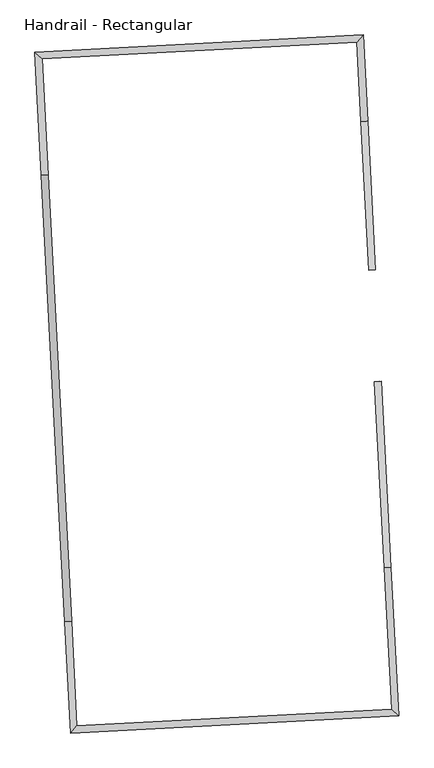
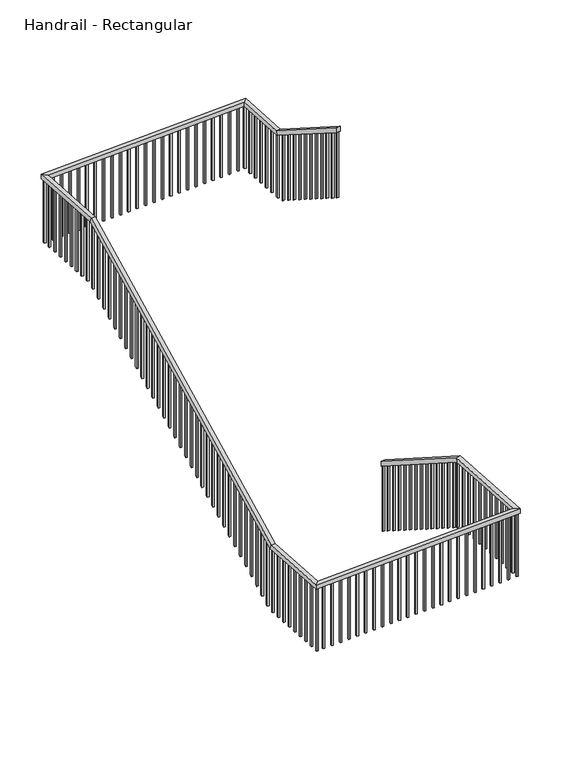
"""IFC4 building model written with IfcOpenShell, lengths in millimetres: railing geometry, Handrail - Rectangular."""

from ifc_helpers import new_model, si_unit, frame, origin, place, context, project, spatial, polyline, outline, extrude, faceted_brep, source, transform, mapped, element, save


def handrail_rectangular_3244dd1d(model_context):
    return source(origin(), model_context, "Body", "SolidModel", [
        faceted_brep([(-3680.4110244, -27041.7227656, 1087.5818182), (-3680.4110244, -27041.7227656, 1027.8146938), (-3731.1414048, -27044.3814322, 1027.8146938), (-3731.1414048, -27044.3814322, 1087.5818182), (-3607.2976935, -28436.8082257, 1953.4909091), (-3606.5405513, -28451.2553599, 1902.6909091), (-3657.2709317, -28453.9140265, 1902.6909091), (-3658.0280739, -28439.4668922, 1953.4909091), (-3548.8070288, -29552.8765937, 1953.4909091), (-3548.8070288, -29552.8765937, 1902.6909091), (-3602.1960758, -29504.8048799, 1902.6909091), (-3602.1960758, -29504.8048799, 1953.4909091), (-6015.5717741, -29682.154256, 1953.4909091), (-6015.5717741, -29682.154256, 1902.6909091), (-5967.5000603, -29628.7652091, 1902.6909091), (-5967.5000603, -29628.7652091, 1953.4909091), (-6283.4324318, -24571.0684342, 3980.8727273), (-6283.4324318, -24571.0684342, 4031.6727273), (-3816.6676865, -24441.7907719, 4031.6727273), (-3816.6676865, -24441.7907719, 3980.8727273), (-6230.0433848, -24619.140148, 3980.8727273), (-3864.7394003, -24495.1798188, 3980.8727273), (-6230.0433848, -24619.140148, 4031.6727273), (-3864.7394003, -24495.1798188, 4031.6727273), (-3782.7696876, -25088.6031215, 4031.6727273), (-3782.0125454, -25103.0502558, 3980.8727273), (-3832.7429258, -25105.7089224, 3980.8727273), (-3833.500068, -25091.2617881, 4031.6727273), (-3724.2790229, -26204.6714896, 4724.4), (-3775.0094033, -26207.3301562, 4724.4), (-3775.0094033, -26207.3301562, 4664.6328756), (-3724.2790229, -26204.6714896, 4664.6328756), (-6059.4397726, -28845.10298, 1953.4909091), (-6060.1969149, -28830.6558457, 1902.6909091), (-6009.4665345, -28827.9971791, 1902.6909091), (-6008.7093923, -28842.4443134, 1953.4909091), (-6234.9117667, -25496.8978759, 4031.6727273), (-6235.6689089, -25482.4507416, 3980.8727273), (-6184.9385286, -25479.792075, 3980.8727273), (-6184.1813864, -25494.2392093, 4031.6727273)], [[[0, 1, 2, 3]], [[1, 0, 4, 5]], [[2, 1, 5, 6]], [[3, 2, 6, 7]], [[0, 3, 7, 4]], [[5, 4, 8, 9]], [[6, 5, 9, 10]], [[7, 6, 10, 11]], [[4, 7, 11, 8]], [[9, 8, 12, 13]], [[10, 9, 13, 14]], [[11, 10, 14, 15]], [[8, 11, 15, 12]], [[16, 17, 18, 19]], [[20, 16, 19, 21]], [[22, 20, 21, 23]], [[17, 22, 23, 18]], [[19, 18, 24, 25]], [[21, 19, 25, 26]], [[23, 21, 26, 27]], [[18, 23, 27, 24]], [[28, 29, 30, 31]], [[25, 24, 28, 31]], [[26, 25, 31, 30]], [[27, 26, 30, 29]], [[24, 27, 29, 28]], [[13, 12, 32, 33]], [[14, 13, 33, 34]], [[15, 14, 34, 35]], [[12, 15, 35, 32]], [[33, 32, 36, 37]], [[34, 33, 37, 38]], [[35, 34, 38, 39]], [[32, 35, 39, 36]], [[37, 36, 17, 16]], [[38, 37, 16, 20]], [[39, 38, 20, 22]], [[36, 39, 22, 17]]]),
        extrude(outline(polyline([(234.5039257, 19.05), (1048.9045305, 19.05), (1037.0966792, 0.0), (222.6960744, 0.0), (234.5039257, 19.05)])), frame((-3763.9749926, -26114.5505084, 4830.257669), z_axis=(0.9986295347545738, 0.052335956242946104, 0.0), x_axis=(0.0, 0.0, -1.0)), (0.0, 0.0, 1.0), 19.05),
        extrude(outline(polyline([(234.5039257, 19.05), (1048.9045305, 19.05), (1037.0966792, 0.0), (222.6960744, 0.0), (234.5039257, 19.05)])), frame((-3769.2923258, -26013.0897477, 4767.2824624), z_axis=(0.9986295347545738, 0.052335956242946104, 0.0), x_axis=(0.0, 0.0, -1.0)), (0.0, 0.0, 1.0), 19.05),
        extrude(outline(polyline([(234.5039256, 19.0500001), (1048.9045304, 19.0500001), (1037.0966791, 0.0), (222.6960743, 0.0), (234.5039256, 19.0500001)])), frame((-3774.6096589, -25911.628987, 4704.3072557), z_axis=(0.9986295347545738, 0.052335956242946104, 0.0), x_axis=(0.0, 0.0, -1.0)), (0.0, 0.0, 1.0), 19.05),
        extrude(outline(polyline([(234.5039256, 19.0500001), (1048.9045304, 19.0500001), (1037.0966792, 0.0), (222.6960744, 0.0), (234.5039256, 19.0500001)])), frame((-3779.9269921, -25810.1682263, 4641.3320491), z_axis=(0.9986295347545738, 0.052335956242946104, 0.0), x_axis=(0.0, 0.0, -1.0)), (0.0, 0.0, 1.0), 19.05),
        extrude(outline(polyline([(234.5039256, 19.05), (1048.9045304, 19.05), (1037.0966792, 0.0), (222.6960744, 0.0), (234.5039256, 19.05)])), frame((-3785.2443252, -25708.7074655, 4578.3568425), z_axis=(0.9986295347545738, 0.052335956242946104, 0.0), x_axis=(0.0, 0.0, -1.0)), (0.0, 0.0, 1.0), 19.05),
        extrude(outline(polyline([(234.5039256, 19.05), (1048.9045304, 19.05), (1037.0966792, 0.0), (222.6960744, 0.0), (234.5039256, 19.05)])), frame((-3790.5616584, -25607.2467048, 4515.3816359), z_axis=(0.9986295347545738, 0.052335956242946104, 0.0), x_axis=(0.0, 0.0, -1.0)), (0.0, 0.0, 1.0), 19.05),
        extrude(outline(polyline([(234.5039256, 19.0500001), (1048.9045304, 19.0500001), (1037.0966792, 0.0), (222.6960744, 0.0), (234.5039256, 19.0500001)])), frame((-3795.8789915, -25505.7859441, 4452.4064293), z_axis=(0.9986295347545738, 0.052335956242946104, 0.0), x_axis=(0.0, 0.0, -1.0)), (0.0, 0.0, 1.0), 19.05),
        extrude(outline(polyline([(234.5039256, 19.05), (1048.9045304, 19.05), (1037.0966792, 0.0), (222.6960744, 0.0), (234.5039256, 19.05)])), frame((-3801.1963247, -25404.3251833, 4389.4312227), z_axis=(0.9986295347545738, 0.052335956242946104, 0.0), x_axis=(0.0, 0.0, -1.0)), (0.0, 0.0, 1.0), 19.05),
        extrude(outline(polyline([(234.5039256, 19.05), (1048.9045305, 19.05), (1037.0966792, 0.0), (222.6960744, 0.0), (234.5039256, 19.05)])), frame((-3806.5136578, -25302.8644226, 4326.4560161), z_axis=(0.9986295347545738, 0.052335956242946104, 0.0), x_axis=(0.0, 0.0, -1.0)), (0.0, 0.0, 1.0), 19.05),
        extrude(outline(polyline([(234.5039257, 19.0500001), (1048.9045305, 19.0500001), (1037.0966792, 0.0), (222.6960744, 0.0), (234.5039257, 19.0500001)])), frame((-3811.830991, -25201.4036619, 4263.4808095), z_axis=(0.9986295347545738, 0.052335956242946104, 0.0), x_axis=(0.0, 0.0, -1.0)), (0.0, 0.0, 1.0), 19.05),
        extrude(outline(polyline([(-3799.7860981, -25067.2394134), (-3798.7890981, -25086.2633061), (-3817.8129908, -25087.260306), (-3818.8099908, -25068.2364134), (-3799.7860981, -25067.2394134)])), frame((0.0, 0.0, 3193.4727273), z_axis=(0.0, 0.0, 1.0), x_axis=(1.0, 0.0, 0.0)), (0.0, 0.0, 1.0), 787.4),
        extrude(outline(polyline([(-3805.1034313, -24965.7786527), (-3804.1064313, -24984.8025453), (-3823.1303239, -24985.7995453), (-3824.1273239, -24966.7756527), (-3805.1034313, -24965.7786527)])), frame((0.0, 0.0, 3193.4727273), z_axis=(0.0, 0.0, 1.0), x_axis=(1.0, 0.0, 0.0)), (0.0, 0.0, 1.0), 787.4),
        extrude(outline(polyline([(-3810.4207644, -24864.317892), (-3809.4237645, -24883.3417846), (-3828.4476571, -24884.3387846), (-3829.4446571, -24865.3148919), (-3810.4207644, -24864.317892)])), frame((0.0, 0.0, 3193.4727273), z_axis=(0.0, 0.0, 1.0), x_axis=(1.0, 0.0, 0.0)), (0.0, 0.0, 1.0), 787.4),
        extrude(outline(polyline([(-3815.7380976, -24762.8571312), (-3814.7410976, -24781.8810239), (-3833.7649902, -24782.8780239), (-3834.7619902, -24763.8541312), (-3815.7380976, -24762.8571312)])), frame((0.0, 0.0, 3193.4727273), z_axis=(0.0, 0.0, 1.0), x_axis=(1.0, 0.0, 0.0)), (0.0, 0.0, 1.0), 787.4),
        extrude(outline(polyline([(-3821.0554307, -24661.3963705), (-3820.0584308, -24680.4202632), (-3839.0823234, -24681.4172631), (-3840.0793234, -24662.3933705), (-3821.0554307, -24661.3963705)])), frame((0.0, 0.0, 3193.4727273), z_axis=(0.0, 0.0, 1.0), x_axis=(1.0, 0.0, 0.0)), (0.0, 0.0, 1.0), 787.4),
        extrude(outline(polyline([(-3826.3727639, -24559.9356098), (-3825.3757639, -24578.9595024), (-3844.3996566, -24579.9565024), (-3845.3966565, -24560.9326098), (-3826.3727639, -24559.9356098)])), frame((0.0, 0.0, 3193.4727273), z_axis=(0.0, 0.0, 1.0), x_axis=(1.0, 0.0, 0.0)), (0.0, 0.0, 1.0), 787.4),
        extrude(outline(polyline([(-3933.1508578, -24463.7921822), (-3914.1269651, -24462.7951822), (-3913.1299652, -24481.8190749), (-3932.1538578, -24482.8160748), (-3933.1508578, -24463.7921822)])), frame((0.0, 0.0, 3193.4727273), z_axis=(0.0, 0.0, 1.0), x_axis=(1.0, 0.0, 0.0)), (0.0, 0.0, 1.0), 787.4),
        extrude(outline(polyline([(-4034.6116185, -24469.1095154), (-4015.5877259, -24468.1125154), (-4014.5907259, -24487.136408), (-4033.6146185, -24488.133408), (-4034.6116185, -24469.1095154)])), frame((0.0, 0.0, 3193.4727273), z_axis=(0.0, 0.0, 1.0), x_axis=(1.0, 0.0, 0.0)), (0.0, 0.0, 1.0), 787.4),
        extrude(outline(polyline([(-4136.0723792, -24474.4268485), (-4117.0484866, -24473.4298486), (-4116.0514866, -24492.4537412), (-4135.0753793, -24493.4507412), (-4136.0723792, -24474.4268485)])), frame((0.0, 0.0, 3193.4727273), z_axis=(0.0, 0.0, 1.0), x_axis=(1.0, 0.0, 0.0)), (0.0, 0.0, 1.0), 787.4),
        extrude(outline(polyline([(-4237.53314, -24479.7441817), (-4218.5092473, -24478.7471817), (-4217.5122474, -24497.7710743), (-4236.53614, -24498.7680743), (-4237.53314, -24479.7441817)])), frame((0.0, 0.0, 3193.4727273), z_axis=(0.0, 0.0, 1.0), x_axis=(1.0, 0.0, 0.0)), (0.0, 0.0, 1.0), 787.4),
        extrude(outline(polyline([(-4338.9939007, -24485.0615148), (-4319.9700081, -24484.0645149), (-4318.9730081, -24503.0884075), (-4337.9969007, -24504.0854075), (-4338.9939007, -24485.0615148)])), frame((0.0, 0.0, 3193.4727273), z_axis=(0.0, 0.0, 1.0), x_axis=(1.0, 0.0, 0.0)), (0.0, 0.0, 1.0), 787.4),
        extrude(outline(polyline([(-4440.4546614, -24490.378848), (-4421.4307688, -24489.381848), (-4420.4337688, -24508.4057407), (-4439.4576615, -24509.4027406), (-4440.4546614, -24490.378848)])), frame((0.0, 0.0, 3193.4727273), z_axis=(0.0, 0.0, 1.0), x_axis=(1.0, 0.0, 0.0)), (0.0, 0.0, 1.0), 787.4),
        extrude(outline(polyline([(-4541.9154222, -24495.6961811), (-4522.8915295, -24494.6991812), (-4521.8945296, -24513.7230738), (-4540.9184222, -24514.7200738), (-4541.9154222, -24495.6961811)])), frame((0.0, 0.0, 3193.4727273), z_axis=(0.0, 0.0, 1.0), x_axis=(1.0, 0.0, 0.0)), (0.0, 0.0, 1.0), 787.4),
        extrude(outline(polyline([(-4643.3761829, -24501.0135143), (-4624.3522903, -24500.0165143), (-4623.3552903, -24519.040407), (-4642.3791829, -24520.0374069), (-4643.3761829, -24501.0135143)])), frame((0.0, 0.0, 3193.4727273), z_axis=(0.0, 0.0, 1.0), x_axis=(1.0, 0.0, 0.0)), (0.0, 0.0, 1.0), 787.4),
        extrude(outline(polyline([(-4744.8369436, -24506.3308474), (-4725.813051, -24505.3338475), (-4724.816051, -24524.3577401), (-4743.8399437, -24525.3547401), (-4744.8369436, -24506.3308474)])), frame((0.0, 0.0, 3193.4727273), z_axis=(0.0, 0.0, 1.0), x_axis=(1.0, 0.0, 0.0)), (0.0, 0.0, 1.0), 787.4),
        extrude(outline(polyline([(-4846.2977044, -24511.6481806), (-4827.2738117, -24510.6511806), (-4826.2768117, -24529.6750733), (-4845.3007044, -24530.6720732), (-4846.2977044, -24511.6481806)])), frame((0.0, 0.0, 3193.4727273), z_axis=(0.0, 0.0, 1.0), x_axis=(1.0, 0.0, 0.0)), (0.0, 0.0, 1.0), 787.4),
        extrude(outline(polyline([(-4947.7584651, -24516.9655138), (-4928.7345724, -24515.9685138), (-4927.7375725, -24534.9924064), (-4946.7614651, -24535.9894064), (-4947.7584651, -24516.9655138)])), frame((0.0, 0.0, 3193.4727273), z_axis=(0.0, 0.0, 1.0), x_axis=(1.0, 0.0, 0.0)), (0.0, 0.0, 1.0), 787.4),
        extrude(outline(polyline([(-5049.2192258, -24522.2828469), (-5030.1953332, -24521.2858469), (-5029.1983332, -24540.3097396), (-5048.2222258, -24541.3067395), (-5049.2192258, -24522.2828469)])), frame((0.0, 0.0, 3193.4727273), z_axis=(0.0, 0.0, 1.0), x_axis=(1.0, 0.0, 0.0)), (0.0, 0.0, 1.0), 787.4),
        extrude(outline(polyline([(-5150.6799865, -24527.6001801), (-5131.6560939, -24526.6031801), (-5130.6590939, -24545.6270727), (-5149.6829866, -24546.6240727), (-5150.6799865, -24527.6001801)])), frame((0.0, 0.0, 3193.4727273), z_axis=(0.0, 0.0, 1.0), x_axis=(1.0, 0.0, 0.0)), (0.0, 0.0, 1.0), 787.4),
        extrude(outline(polyline([(-5252.1407473, -24532.9175132), (-5233.1168546, -24531.9205132), (-5232.1198547, -24550.9444059), (-5251.1437473, -24551.9414059), (-5252.1407473, -24532.9175132)])), frame((0.0, 0.0, 3193.4727273), z_axis=(0.0, 0.0, 1.0), x_axis=(1.0, 0.0, 0.0)), (0.0, 0.0, 1.0), 787.4),
        extrude(outline(polyline([(-5353.601508, -24538.2348464), (-5334.5776154, -24537.2378464), (-5333.5806154, -24556.261739), (-5352.604508, -24557.258739), (-5353.601508, -24538.2348464)])), frame((0.0, 0.0, 3193.4727273), z_axis=(0.0, 0.0, 1.0), x_axis=(1.0, 0.0, 0.0)), (0.0, 0.0, 1.0), 787.4),
        extrude(outline(polyline([(-5455.0622687, -24543.5521795), (-5436.0383761, -24542.5551796), (-5435.0413761, -24561.5790722), (-5454.0652688, -24562.5760722), (-5455.0622687, -24543.5521795)])), frame((0.0, 0.0, 3193.4727273), z_axis=(0.0, 0.0, 1.0), x_axis=(1.0, 0.0, 0.0)), (0.0, 0.0, 1.0), 787.4),
        extrude(outline(polyline([(-5556.5230295, -24548.8695127), (-5537.4991368, -24547.8725127), (-5536.5021369, -24566.8964053), (-5555.5260295, -24567.8934053), (-5556.5230295, -24548.8695127)])), frame((0.0, 0.0, 3193.4727273), z_axis=(0.0, 0.0, 1.0), x_axis=(1.0, 0.0, 0.0)), (0.0, 0.0, 1.0), 787.4),
        extrude(outline(polyline([(-5657.9837902, -24554.1868458), (-5638.9598976, -24553.1898459), (-5637.9628976, -24572.2137385), (-5656.9867902, -24573.2107385), (-5657.9837902, -24554.1868458)])), frame((0.0, 0.0, 3193.4727273), z_axis=(0.0, 0.0, 1.0), x_axis=(1.0, 0.0, 0.0)), (0.0, 0.0, 1.0), 787.4),
        extrude(outline(polyline([(-5759.4445509, -24559.504179), (-5740.4206583, -24558.507179), (-5739.4236583, -24577.5310717), (-5758.447551, -24578.5280716), (-5759.4445509, -24559.504179)])), frame((0.0, 0.0, 3193.4727273), z_axis=(0.0, 0.0, 1.0), x_axis=(1.0, 0.0, 0.0)), (0.0, 0.0, 1.0), 787.4),
        extrude(outline(polyline([(-5860.9053117, -24564.8215121), (-5841.881419, -24563.8245122), (-5840.8844191, -24582.8484048), (-5859.9083117, -24583.8454048), (-5860.9053117, -24564.8215121)])), frame((0.0, 0.0, 3193.4727273), z_axis=(0.0, 0.0, 1.0), x_axis=(1.0, 0.0, 0.0)), (0.0, 0.0, 1.0), 787.4),
        extrude(outline(polyline([(-5962.3660724, -24570.1388453), (-5943.3421798, -24569.1418453), (-5942.3451798, -24588.165738), (-5961.3690724, -24589.1627379), (-5962.3660724, -24570.1388453)])), frame((0.0, 0.0, 3193.4727273), z_axis=(0.0, 0.0, 1.0), x_axis=(1.0, 0.0, 0.0)), (0.0, 0.0, 1.0), 787.4),
        extrude(outline(polyline([(-6063.8268331, -24575.4561784), (-6044.8029405, -24574.4591785), (-6043.8059405, -24593.4830711), (-6062.8298332, -24594.4800711), (-6063.8268331, -24575.4561784)])), frame((0.0, 0.0, 3193.4727273), z_axis=(0.0, 0.0, 1.0), x_axis=(1.0, 0.0, 0.0)), (0.0, 0.0, 1.0), 787.4),
        extrude(outline(polyline([(-6165.2875939, -24580.7735116), (-6146.2637012, -24579.7765116), (-6145.2667013, -24598.8004043), (-6164.2905939, -24599.7974042), (-6165.2875939, -24580.7735116)])), frame((0.0, 0.0, 3193.4727273), z_axis=(0.0, 0.0, 1.0), x_axis=(1.0, 0.0, 0.0)), (0.0, 0.0, 1.0), 787.4),
        extrude(outline(polyline([(-6261.0986881, -24693.892903), (-6262.0956881, -24674.8690104), (-6243.0717954, -24673.8720104), (-6242.0747955, -24692.8959031), (-6261.0986881, -24693.892903)])), frame((0.0, 0.0, 3193.4727273), z_axis=(0.0, 0.0, 1.0), x_axis=(1.0, 0.0, 0.0)), (0.0, 0.0, 1.0), 787.4),
        extrude(outline(polyline([(-6255.781355, -24795.3536638), (-6256.7783549, -24776.3297711), (-6237.7544623, -24775.3327712), (-6236.7574623, -24794.3566638), (-6255.781355, -24795.3536638)])), frame((0.0, 0.0, 3193.4727273), z_axis=(0.0, 0.0, 1.0), x_axis=(1.0, 0.0, 0.0)), (0.0, 0.0, 1.0), 787.4),
        extrude(outline(polyline([(-6250.4640218, -24896.8144245), (-6251.4610218, -24877.7905319), (-6232.4371291, -24876.7935319), (-6231.4401292, -24895.8174245), (-6250.4640218, -24896.8144245)])), frame((0.0, 0.0, 3193.4727273), z_axis=(0.0, 0.0, 1.0), x_axis=(1.0, 0.0, 0.0)), (0.0, 0.0, 1.0), 787.4),
        extrude(outline(polyline([(-6245.1466886, -24998.2751852), (-6246.1436886, -24979.2512926), (-6227.119796, -24978.2542926), (-6226.122796, -24997.2781853), (-6245.1466886, -24998.2751852)])), frame((0.0, 0.0, 3193.4727273), z_axis=(0.0, 0.0, 1.0), x_axis=(1.0, 0.0, 0.0)), (0.0, 0.0, 1.0), 787.4),
        extrude(outline(polyline([(-6239.8293555, -25099.735946), (-6240.8263555, -25080.7120533), (-6221.8024628, -25079.7150534), (-6220.8054629, -25098.738946), (-6239.8293555, -25099.735946)])), frame((0.0, 0.0, 3193.4727273), z_axis=(0.0, 0.0, 1.0), x_axis=(1.0, 0.0, 0.0)), (0.0, 0.0, 1.0), 787.4),
        extrude(outline(polyline([(-6234.5120223, -25201.1967067), (-6235.5090223, -25182.1728141), (-6216.4851297, -25181.1758141), (-6215.4881297, -25200.1997067), (-6234.5120223, -25201.1967067)])), frame((0.0, 0.0, 3193.4727273), z_axis=(0.0, 0.0, 1.0), x_axis=(1.0, 0.0, 0.0)), (0.0, 0.0, 1.0), 787.4),
        extrude(outline(polyline([(-6229.1946892, -25302.6574674), (-6230.1916892, -25283.6335748), (-6211.1677965, -25282.6365748), (-6210.1707965, -25301.6604675), (-6229.1946892, -25302.6574674)])), frame((0.0, 0.0, 3193.4727273), z_axis=(0.0, 0.0, 1.0), x_axis=(1.0, 0.0, 0.0)), (0.0, 0.0, 1.0), 787.4),
        extrude(outline(polyline([(-6223.877356, -25404.1182282), (-6224.874356, -25385.0943355), (-6205.8504634, -25384.0973355), (-6204.8534634, -25403.1212282), (-6223.877356, -25404.1182282)])), frame((0.0, 0.0, 3193.4727273), z_axis=(0.0, 0.0, 1.0), x_axis=(1.0, 0.0, 0.0)), (0.0, 0.0, 1.0), 787.4),
        extrude(outline(polyline([(222.6960743, 19.05), (1037.0966792, 19.05), (1048.9045304, 0.0), (234.5039256, 0.0), (222.6960743, 19.05)])), frame((-6213.2426897, -25607.0397496, 4137.5303962), z_axis=(0.9986295347545738, 0.052335956242946104, 0.0), x_axis=(0.0, 0.0, -1.0)), (0.0, 0.0, 1.0), 19.05),
        extrude(outline(polyline([(222.6960744, 19.05), (1037.0966792, 19.05), (1048.9045304, 0.0), (234.5039256, 0.0), (222.6960744, 19.05)])), frame((-6207.9253566, -25708.5005103, 4074.5551896), z_axis=(0.9986295347545738, 0.052335956242946104, 0.0), x_axis=(0.0, 0.0, -1.0)), (0.0, 0.0, 1.0), 19.05),
        extrude(outline(polyline([(222.6960744, 19.0500001), (1037.0966792, 19.0500001), (1048.9045304, 0.0), (234.5039256, 0.0), (222.6960744, 19.0500001)])), frame((-6202.6080234, -25809.9612711, 4011.579983), z_axis=(0.9986295347545738, 0.052335956242946104, 0.0), x_axis=(0.0, 0.0, -1.0)), (0.0, 0.0, 1.0), 19.05),
        extrude(outline(polyline([(222.6960744, 19.05), (1037.0966792, 19.05), (1048.9045304, 0.0), (234.5039256, 0.0), (222.6960744, 19.05)])), frame((-6197.2906903, -25911.4220318, 3948.6047764), z_axis=(0.9986295347545738, 0.052335956242946104, 0.0), x_axis=(0.0, 0.0, -1.0)), (0.0, 0.0, 1.0), 19.05),
        extrude(outline(polyline([(222.6960744, 19.05), (1037.0966792, 19.05), (1048.9045304, 0.0), (234.5039256, 0.0), (222.6960744, 19.05)])), frame((-6191.9733571, -26012.8827925, 3885.6295698), z_axis=(0.9986295347545738, 0.052335956242946104, 0.0), x_axis=(0.0, 0.0, -1.0)), (0.0, 0.0, 1.0), 19.05),
        extrude(outline(polyline([(222.6960744, 19.0500001), (1037.0966792, 19.0500001), (1048.9045304, 0.0), (234.5039256, 0.0), (222.6960744, 19.0500001)])), frame((-6186.656024, -26114.3435533, 3822.6543632), z_axis=(0.9986295347545738, 0.052335956242946104, 0.0), x_axis=(0.0, 0.0, -1.0)), (0.0, 0.0, 1.0), 19.05),
        extrude(outline(polyline([(222.6960744, 19.05), (1037.0966792, 19.05), (1048.9045305, 0.0), (234.5039257, 0.0), (222.6960744, 19.05)])), frame((-6181.3386908, -26215.804314, 3759.6791566), z_axis=(0.9986295347545738, 0.052335956242946104, 0.0), x_axis=(0.0, 0.0, -1.0)), (0.0, 0.0, 1.0), 19.05),
        extrude(outline(polyline([(222.6960744, 19.05), (1037.0966792, 19.05), (1048.9045305, 0.0), (234.5039257, 0.0), (222.6960744, 19.05)])), frame((-6176.0213576, -26317.2650747, 3696.70395), z_axis=(0.9986295347545738, 0.052335956242946104, 0.0), x_axis=(0.0, 0.0, -1.0)), (0.0, 0.0, 1.0), 19.05),
        extrude(outline(polyline([(222.6960743, 19.0500001), (1037.0966791, 19.0500001), (1048.9045304, 0.0), (234.5039256, 0.0), (222.6960743, 19.0500001)])), frame((-6170.7040245, -26418.7258355, 3633.7287433), z_axis=(0.9986295347545738, 0.052335956242946104, 0.0), x_axis=(0.0, 0.0, -1.0)), (0.0, 0.0, 1.0), 19.05),
        extrude(outline(polyline([(222.6960743, 19.05), (1037.0966792, 19.05), (1048.9045304, 0.0), (234.5039256, 0.0), (222.6960743, 19.05)])), frame((-6165.3866913, -26520.1865962, 3570.7535367), z_axis=(0.9986295347545738, 0.052335956242946104, 0.0), x_axis=(0.0, 0.0, -1.0)), (0.0, 0.0, 1.0), 19.05),
        extrude(outline(polyline([(222.6960744, 19.05), (1037.0966792, 19.05), (1048.9045304, 0.0), (234.5039256, 0.0), (222.6960744, 19.05)])), frame((-6160.0693582, -26621.6473569, 3507.7783301), z_axis=(0.9986295347545738, 0.052335956242946104, 0.0), x_axis=(0.0, 0.0, -1.0)), (0.0, 0.0, 1.0), 19.05),
        extrude(outline(polyline([(222.6960744, 19.0500001), (1037.0966792, 19.0500001), (1048.9045304, 0.0), (234.5039256, 0.0), (222.6960744, 19.0500001)])), frame((-6154.752025, -26723.1081177, 3444.8031235), z_axis=(0.9986295347545738, 0.052335956242946104, 0.0), x_axis=(0.0, 0.0, -1.0)), (0.0, 0.0, 1.0), 19.05),
        extrude(outline(polyline([(222.6960744, 19.0500001), (1037.0966792, 19.0500001), (1048.9045304, 0.0), (234.5039256, 0.0), (222.6960744, 19.0500001)])), frame((-6149.4346919, -26824.5688784, 3381.8279169), z_axis=(0.9986295347545738, 0.052335956242946104, 0.0), x_axis=(0.0, 0.0, -1.0)), (0.0, 0.0, 1.0), 19.05),
        extrude(outline(polyline([(222.6960744, 19.05), (1037.0966792, 19.05), (1048.9045304, 0.0), (234.5039256, 0.0), (222.6960744, 19.05)])), frame((-6144.1173587, -26926.0296391, 3318.8527103), z_axis=(0.9986295347545738, 0.052335956242946104, 0.0), x_axis=(0.0, 0.0, -1.0)), (0.0, 0.0, 1.0), 19.05),
        extrude(outline(polyline([(222.6960744, 19.05), (1037.0966792, 19.05), (1048.9045305, 0.0), (234.5039256, 0.0), (222.6960744, 19.05)])), frame((-6138.8000256, -27027.4903998, 3255.8775037), z_axis=(0.9986295347545738, 0.052335956242946104, 0.0), x_axis=(0.0, 0.0, -1.0)), (0.0, 0.0, 1.0), 19.05),
        extrude(outline(polyline([(222.6960744, 19.0500001), (1037.0966792, 19.0500001), (1048.9045305, 0.0), (234.5039257, 0.0), (222.6960744, 19.0500001)])), frame((-6133.4826924, -27128.9511606, 3192.9022971), z_axis=(0.9986295347545738, 0.052335956242946104, 0.0), x_axis=(0.0, 0.0, -1.0)), (0.0, 0.0, 1.0), 19.05),
        extrude(outline(polyline([(222.6960744, 19.05), (1037.0966792, 19.05), (1048.9045305, 0.0), (234.5039257, 0.0), (222.6960744, 19.05)])), frame((-6128.1653593, -27230.4119213, 3129.9270905), z_axis=(0.9986295347545738, 0.052335956242946104, 0.0), x_axis=(0.0, 0.0, -1.0)), (0.0, 0.0, 1.0), 19.05),
        extrude(outline(polyline([(222.6960743, 19.05), (1037.0966791, 19.05), (1048.9045304, 0.0), (234.5039256, 0.0), (222.6960743, 19.05)])), frame((-6122.8480261, -27331.872682, 3066.9518838), z_axis=(0.9986295347545738, 0.052335956242946104, 0.0), x_axis=(0.0, 0.0, -1.0)), (0.0, 0.0, 1.0), 19.05),
        extrude(outline(polyline([(222.6960744, 19.0500001), (1037.0966792, 19.0500001), (1048.9045304, 0.0), (234.5039256, 0.0), (222.6960744, 19.0500001)])), frame((-6117.5306929, -27433.3334428, 3003.9766772), z_axis=(0.9986295347545738, 0.052335956242946104, 0.0), x_axis=(0.0, 0.0, -1.0)), (0.0, 0.0, 1.0), 19.05),
        extrude(outline(polyline([(222.6960744, 19.05), (1037.0966792, 19.05), (1048.9045304, 0.0), (234.5039256, 0.0), (222.6960744, 19.05)])), frame((-6112.2133598, -27534.7942035, 2941.0014706), z_axis=(0.9986295347545738, 0.052335956242946104, 0.0), x_axis=(0.0, 0.0, -1.0)), (0.0, 0.0, 1.0), 19.05),
        extrude(outline(polyline([(222.6960744, 19.05), (1037.0966792, 19.05), (1048.9045304, 0.0), (234.5039256, 0.0), (222.6960744, 19.05)])), frame((-6106.8960266, -27636.2549642, 2878.026264), z_axis=(0.9986295347545738, 0.052335956242946104, 0.0), x_axis=(0.0, 0.0, -1.0)), (0.0, 0.0, 1.0), 19.05),
        extrude(outline(polyline([(222.6960744, 19.0500001), (1037.0966792, 19.0500001), (1048.9045304, 0.0), (234.5039256, 0.0), (222.6960744, 19.0500001)])), frame((-6101.5786935, -27737.715725, 2815.0510574), z_axis=(0.9986295347545738, 0.052335956242946104, 0.0), x_axis=(0.0, 0.0, -1.0)), (0.0, 0.0, 1.0), 19.05),
        extrude(outline(polyline([(222.6960744, 19.05), (1037.0966792, 19.05), (1048.9045304, 0.0), (234.5039256, 0.0), (222.6960744, 19.05)])), frame((-6096.2613603, -27839.1764857, 2752.0758508), z_axis=(0.9986295347545738, 0.052335956242946104, 0.0), x_axis=(0.0, 0.0, -1.0)), (0.0, 0.0, 1.0), 19.05),
        extrude(outline(polyline([(222.6960744, 19.05), (1037.0966792, 19.05), (1048.9045305, 0.0), (234.5039256, 0.0), (222.6960744, 19.05)])), frame((-6090.9440272, -27940.6372464, 2689.1006442), z_axis=(0.9986295347545738, 0.052335956242946104, 0.0), x_axis=(0.0, 0.0, -1.0)), (0.0, 0.0, 1.0), 19.05),
        extrude(outline(polyline([(222.6960744, 19.0500001), (1037.0966792, 19.0500001), (1048.9045305, 0.0), (234.5039257, 0.0), (222.6960744, 19.0500001)])), frame((-6085.626694, -28042.0980072, 2626.1254376), z_axis=(0.9986295347545738, 0.052335956242946104, 0.0), x_axis=(0.0, 0.0, -1.0)), (0.0, 0.0, 1.0), 19.05),
        extrude(outline(polyline([(222.6960743, 19.05), (1037.0966791, 19.05), (1048.9045304, 0.0), (234.5039256, 0.0), (222.6960743, 19.05)])), frame((-6080.3093609, -28143.5587679, 2563.1502309), z_axis=(0.9986295347545738, 0.052335956242946104, 0.0), x_axis=(0.0, 0.0, -1.0)), (0.0, 0.0, 1.0), 19.05),
        extrude(outline(polyline([(222.6960743, 19.05), (1037.0966792, 19.05), (1048.9045304, 0.0), (234.5039256, 0.0), (222.6960743, 19.05)])), frame((-6074.9920277, -28245.0195286, 2500.1750243), z_axis=(0.9986295347545738, 0.052335956242946104, 0.0), x_axis=(0.0, 0.0, -1.0)), (0.0, 0.0, 1.0), 19.05),
        extrude(outline(polyline([(222.6960744, 19.0500001), (1037.0966792, 19.0500001), (1048.9045304, 0.0), (234.5039256, 0.0), (222.6960744, 19.0500001)])), frame((-6069.6746946, -28346.4802894, 2437.1998177), z_axis=(0.9986295347545738, 0.052335956242946104, 0.0), x_axis=(0.0, 0.0, -1.0)), (0.0, 0.0, 1.0), 19.05),
        extrude(outline(polyline([(222.6960744, 19.0500001), (1037.0966792, 19.0500001), (1048.9045304, 0.0), (234.5039256, 0.0), (222.6960744, 19.0500001)])), frame((-6064.3573614, -28447.9410501, 2374.2246111), z_axis=(0.9986295347545738, 0.052335956242946104, 0.0), x_axis=(0.0, 0.0, -1.0)), (0.0, 0.0, 1.0), 19.05),
        extrude(outline(polyline([(222.6960744, 19.05), (1037.0966792, 19.05), (1048.9045304, 0.0), (234.5039256, 0.0), (222.6960744, 19.05)])), frame((-6059.0400282, -28549.4018108, 2311.2494045), z_axis=(0.9986295347545738, 0.052335956242946104, 0.0), x_axis=(0.0, 0.0, -1.0)), (0.0, 0.0, 1.0), 19.05),
        extrude(outline(polyline([(222.6960744, 19.05), (1037.0966792, 19.05), (1048.9045304, 0.0), (234.5039256, 0.0), (222.6960744, 19.05)])), frame((-6053.7226951, -28650.8625715, 2248.2741979), z_axis=(0.9986295347545738, 0.052335956242946104, 0.0), x_axis=(0.0, 0.0, -1.0)), (0.0, 0.0, 1.0), 19.05),
        extrude(outline(polyline([(222.6960744, 19.0500001), (1037.0966792, 19.0500001), (1048.9045305, 0.0), (234.5039256, 0.0), (222.6960744, 19.0500001)])), frame((-6048.4053619, -28752.3233323, 2185.2989913), z_axis=(0.9986295347545738, 0.052335956242946104, 0.0), x_axis=(0.0, 0.0, -1.0)), (0.0, 0.0, 1.0), 19.05),
        extrude(outline(polyline([(-6037.7706956, -28955.2448537), (-6038.7676956, -28936.2209611), (-6019.743803, -28935.2239611), (-6018.746803, -28954.2478538), (-6037.7706956, -28955.2448537)])), frame((0.0, 0.0, 1115.2909091), z_axis=(0.0, 0.0, 1.0), x_axis=(1.0, 0.0, 0.0)), (0.0, 0.0, 1.0), 787.4),
        extrude(outline(polyline([(-6032.4533625, -29056.7056145), (-6033.4503624, -29037.6817218), (-6014.4264698, -29036.6847219), (-6013.4294698, -29055.7086145), (-6032.4533625, -29056.7056145)])), frame((0.0, 0.0, 1115.2909091), z_axis=(0.0, 0.0, 1.0), x_axis=(1.0, 0.0, 0.0)), (0.0, 0.0, 1.0), 787.4),
        extrude(outline(polyline([(-6027.1360293, -29158.1663752), (-6028.1330293, -29139.1424826), (-6009.1091367, -29138.1454826), (-6008.1121367, -29157.1693752), (-6027.1360293, -29158.1663752)])), frame((0.0, 0.0, 1115.2909091), z_axis=(0.0, 0.0, 1.0), x_axis=(1.0, 0.0, 0.0)), (0.0, 0.0, 1.0), 787.4),
        extrude(outline(polyline([(-6021.8186962, -29259.6271359), (-6022.8156961, -29240.6032433), (-6003.7918035, -29239.6062433), (-6002.7948035, -29258.630136), (-6021.8186962, -29259.6271359)])), frame((0.0, 0.0, 1115.2909091), z_axis=(0.0, 0.0, 1.0), x_axis=(1.0, 0.0, 0.0)), (0.0, 0.0, 1.0), 787.4),
        extrude(outline(polyline([(-6016.501363, -29361.0878967), (-6017.498363, -29342.064004), (-5998.4744703, -29341.0670041), (-5997.4774704, -29360.0908967), (-6016.501363, -29361.0878967)])), frame((0.0, 0.0, 1115.2909091), z_axis=(0.0, 0.0, 1.0), x_axis=(1.0, 0.0, 0.0)), (0.0, 0.0, 1.0), 787.4),
        extrude(outline(polyline([(-6011.1840299, -29462.5486574), (-6012.1810298, -29443.5247648), (-5993.1571372, -29442.5277648), (-5992.1601372, -29461.5516574), (-6011.1840299, -29462.5486574)])), frame((0.0, 0.0, 1115.2909091), z_axis=(0.0, 0.0, 1.0), x_axis=(1.0, 0.0, 0.0)), (0.0, 0.0, 1.0), 787.4),
        extrude(outline(polyline([(-6005.8666967, -29564.0094181), (-6006.8636967, -29544.9855255), (-5987.839804, -29543.9885255), (-5986.8428041, -29563.0124182), (-6005.8666967, -29564.0094181)])), frame((0.0, 0.0, 1115.2909091), z_axis=(0.0, 0.0, 1.0), x_axis=(1.0, 0.0, 0.0)), (0.0, 0.0, 1.0), 787.4),
        extrude(outline(polyline([(-5899.0886028, -29660.1528457), (-5918.1124955, -29661.1498457), (-5919.1094954, -29642.125953), (-5900.0856028, -29641.1289531), (-5899.0886028, -29660.1528457)])), frame((0.0, 0.0, 1115.2909091), z_axis=(0.0, 0.0, 1.0), x_axis=(1.0, 0.0, 0.0)), (0.0, 0.0, 1.0), 787.4),
        extrude(outline(polyline([(-5797.6278421, -29654.8355125), (-5816.6517347, -29655.8325125), (-5817.6487347, -29636.8086199), (-5798.6248421, -29635.8116199), (-5797.6278421, -29654.8355125)])), frame((0.0, 0.0, 1115.2909091), z_axis=(0.0, 0.0, 1.0), x_axis=(1.0, 0.0, 0.0)), (0.0, 0.0, 1.0), 787.4),
        extrude(outline(polyline([(-5696.1670814, -29649.5181794), (-5715.190974, -29650.5151794), (-5716.187974, -29631.4912867), (-5697.1640813, -29630.4942868), (-5696.1670814, -29649.5181794)])), frame((0.0, 0.0, 1115.2909091), z_axis=(0.0, 0.0, 1.0), x_axis=(1.0, 0.0, 0.0)), (0.0, 0.0, 1.0), 787.4),
        extrude(outline(polyline([(-5594.7063206, -29644.2008462), (-5613.7302133, -29645.1978462), (-5614.7272132, -29626.1739536), (-5595.7033206, -29625.1769536), (-5594.7063206, -29644.2008462)])), frame((0.0, 0.0, 1115.2909091), z_axis=(0.0, 0.0, 1.0), x_axis=(1.0, 0.0, 0.0)), (0.0, 0.0, 1.0), 787.4),
        extrude(outline(polyline([(-5493.2455599, -29638.8835131), (-5512.2694525, -29639.8805131), (-5513.2664525, -29620.8566204), (-5494.2425599, -29619.8596204), (-5493.2455599, -29638.8835131)])), frame((0.0, 0.0, 1115.2909091), z_axis=(0.0, 0.0, 1.0), x_axis=(1.0, 0.0, 0.0)), (0.0, 0.0, 1.0), 787.4),
        extrude(outline(polyline([(-5391.7847992, -29633.5661799), (-5410.8086918, -29634.5631799), (-5411.8056918, -29615.5392873), (-5392.7817991, -29614.5422873), (-5391.7847992, -29633.5661799)])), frame((0.0, 0.0, 1115.2909091), z_axis=(0.0, 0.0, 1.0), x_axis=(1.0, 0.0, 0.0)), (0.0, 0.0, 1.0), 787.4),
        extrude(outline(polyline([(-5290.3240384, -29628.2488468), (-5309.3479311, -29629.2458467), (-5310.344931, -29610.2219541), (-5291.3210384, -29609.2249541), (-5290.3240384, -29628.2488468)])), frame((0.0, 0.0, 1115.2909091), z_axis=(0.0, 0.0, 1.0), x_axis=(1.0, 0.0, 0.0)), (0.0, 0.0, 1.0), 787.4),
        extrude(outline(polyline([(-5188.8632777, -29622.9315136), (-5207.8871703, -29623.9285136), (-5208.8841703, -29604.904621), (-5189.8602777, -29603.907621), (-5188.8632777, -29622.9315136)])), frame((0.0, 0.0, 1115.2909091), z_axis=(0.0, 0.0, 1.0), x_axis=(1.0, 0.0, 0.0)), (0.0, 0.0, 1.0), 787.4),
        extrude(outline(polyline([(-5087.402517, -29617.6141805), (-5106.4264096, -29618.6111804), (-5107.4234096, -29599.5872878), (-5088.3995169, -29598.5902878), (-5087.402517, -29617.6141805)])), frame((0.0, 0.0, 1115.2909091), z_axis=(0.0, 0.0, 1.0), x_axis=(1.0, 0.0, 0.0)), (0.0, 0.0, 1.0), 787.4),
        extrude(outline(polyline([(-4985.9417562, -29612.2968473), (-5004.9656489, -29613.2938473), (-5005.9626488, -29594.2699546), (-4986.9387562, -29593.2729547), (-4985.9417562, -29612.2968473)])), frame((0.0, 0.0, 1115.2909091), z_axis=(0.0, 0.0, 1.0), x_axis=(1.0, 0.0, 0.0)), (0.0, 0.0, 1.0), 787.4),
        extrude(outline(polyline([(-4884.4809955, -29606.9795142), (-4903.5048881, -29607.9765141), (-4904.5018881, -29588.9526215), (-4885.4779955, -29587.9556215), (-4884.4809955, -29606.9795142)])), frame((0.0, 0.0, 1115.2909091), z_axis=(0.0, 0.0, 1.0), x_axis=(1.0, 0.0, 0.0)), (0.0, 0.0, 1.0), 787.4),
        extrude(outline(polyline([(-4783.0202348, -29601.662181), (-4802.0441274, -29602.659181), (-4803.0411274, -29583.6352883), (-4784.0172347, -29582.6382884), (-4783.0202348, -29601.662181)])), frame((0.0, 0.0, 1115.2909091), z_axis=(0.0, 0.0, 1.0), x_axis=(1.0, 0.0, 0.0)), (0.0, 0.0, 1.0), 787.4),
        extrude(outline(polyline([(-4681.559474, -29596.3448479), (-4700.5833667, -29597.3418478), (-4701.5803667, -29578.3179552), (-4682.556474, -29577.3209552), (-4681.559474, -29596.3448479)])), frame((0.0, 0.0, 1115.2909091), z_axis=(0.0, 0.0, 1.0), x_axis=(1.0, 0.0, 0.0)), (0.0, 0.0, 1.0), 787.4),
        extrude(outline(polyline([(-4580.0987133, -29591.0275147), (-4599.122606, -29592.0245147), (-4600.1196059, -29573.000622), (-4581.0957133, -29572.0036221), (-4580.0987133, -29591.0275147)])), frame((0.0, 0.0, 1115.2909091), z_axis=(0.0, 0.0, 1.0), x_axis=(1.0, 0.0, 0.0)), (0.0, 0.0, 1.0), 787.4),
        extrude(outline(polyline([(-4478.6379526, -29585.7101815), (-4497.6618452, -29586.7071815), (-4498.6588452, -29567.6832889), (-4479.6349526, -29566.6862889), (-4478.6379526, -29585.7101815)])), frame((0.0, 0.0, 1115.2909091), z_axis=(0.0, 0.0, 1.0), x_axis=(1.0, 0.0, 0.0)), (0.0, 0.0, 1.0), 787.4),
        extrude(outline(polyline([(-4377.1771919, -29580.3928484), (-4396.2010845, -29581.3898484), (-4397.1980845, -29562.3659557), (-4378.1741918, -29561.3689558), (-4377.1771919, -29580.3928484)])), frame((0.0, 0.0, 1115.2909091), z_axis=(0.0, 0.0, 1.0), x_axis=(1.0, 0.0, 0.0)), (0.0, 0.0, 1.0), 787.4),
        extrude(outline(polyline([(-4275.7164311, -29575.0755152), (-4294.7403238, -29576.0725152), (-4295.7373237, -29557.0486226), (-4276.7134311, -29556.0516226), (-4275.7164311, -29575.0755152)])), frame((0.0, 0.0, 1115.2909091), z_axis=(0.0, 0.0, 1.0), x_axis=(1.0, 0.0, 0.0)), (0.0, 0.0, 1.0), 787.4),
        extrude(outline(polyline([(-4174.2556704, -29569.7581821), (-4193.279563, -29570.755182), (-4194.276563, -29551.7312894), (-4175.2526704, -29550.7342894), (-4174.2556704, -29569.7581821)])), frame((0.0, 0.0, 1115.2909091), z_axis=(0.0, 0.0, 1.0), x_axis=(1.0, 0.0, 0.0)), (0.0, 0.0, 1.0), 787.4),
        extrude(outline(polyline([(-4072.7949097, -29564.4408489), (-4091.8188023, -29565.4378489), (-4092.8158023, -29546.4139563), (-4073.7919096, -29545.4169563), (-4072.7949097, -29564.4408489)])), frame((0.0, 0.0, 1115.2909091), z_axis=(0.0, 0.0, 1.0), x_axis=(1.0, 0.0, 0.0)), (0.0, 0.0, 1.0), 787.4),
        extrude(outline(polyline([(-3971.3341489, -29559.1235158), (-3990.3580416, -29560.1205157), (-3991.3550415, -29541.0966231), (-3972.3311489, -29540.0996231), (-3971.3341489, -29559.1235158)])), frame((0.0, 0.0, 1115.2909091), z_axis=(0.0, 0.0, 1.0), x_axis=(1.0, 0.0, 0.0)), (0.0, 0.0, 1.0), 787.4),
        extrude(outline(polyline([(-3869.8733882, -29553.8061826), (-3888.8972808, -29554.8031826), (-3889.8942808, -29535.7792899), (-3870.8703882, -29534.78229), (-3869.8733882, -29553.8061826)])), frame((0.0, 0.0, 1115.2909091), z_axis=(0.0, 0.0, 1.0), x_axis=(1.0, 0.0, 0.0)), (0.0, 0.0, 1.0), 787.4),
        extrude(outline(polyline([(-3768.4126275, -29548.4888495), (-3787.4365201, -29549.4858494), (-3788.4335201, -29530.4619568), (-3769.4096274, -29529.4649568), (-3768.4126275, -29548.4888495)])), frame((0.0, 0.0, 1115.2909091), z_axis=(0.0, 0.0, 1.0), x_axis=(1.0, 0.0, 0.0)), (0.0, 0.0, 1.0), 787.4),
        extrude(outline(polyline([(-3666.9518667, -29543.1715163), (-3685.9757594, -29544.1685163), (-3686.9727593, -29525.1446236), (-3667.9488667, -29524.1476237), (-3666.9518667, -29543.1715163)])), frame((0.0, 0.0, 1115.2909091), z_axis=(0.0, 0.0, 1.0), x_axis=(1.0, 0.0, 0.0)), (0.0, 0.0, 1.0), 787.4),
        extrude(outline(polyline([(-3570.4761058, -29442.73472), (-3569.4791059, -29461.7586126), (-3588.5029985, -29462.7556126), (-3589.4999985, -29443.7317199), (-3570.4761058, -29442.73472)])), frame((0.0, 0.0, 1115.2909091), z_axis=(0.0, 0.0, 1.0), x_axis=(1.0, 0.0, 0.0)), (0.0, 0.0, 1.0), 787.4),
        extrude(outline(polyline([(-3575.793439, -29341.2739592), (-3574.796439, -29360.2978519), (-3593.8203317, -29361.2948518), (-3594.8173316, -29342.2709592), (-3575.793439, -29341.2739592)])), frame((0.0, 0.0, 1115.2909091), z_axis=(0.0, 0.0, 1.0), x_axis=(1.0, 0.0, 0.0)), (0.0, 0.0, 1.0), 787.4),
        extrude(outline(polyline([(-3581.1107721, -29239.8131985), (-3580.1137722, -29258.8370911), (-3599.1376648, -29259.8340911), (-3600.1346648, -29240.8101985), (-3581.1107721, -29239.8131985)])), frame((0.0, 0.0, 1115.2909091), z_axis=(0.0, 0.0, 1.0), x_axis=(1.0, 0.0, 0.0)), (0.0, 0.0, 1.0), 787.4),
        extrude(outline(polyline([(-3586.4281053, -29138.3524378), (-3585.4311053, -29157.3763304), (-3604.454998, -29158.3733304), (-3605.4519979, -29139.3494377), (-3586.4281053, -29138.3524378)])), frame((0.0, 0.0, 1115.2909091), z_axis=(0.0, 0.0, 1.0), x_axis=(1.0, 0.0, 0.0)), (0.0, 0.0, 1.0), 787.4),
        extrude(outline(polyline([(-3591.7454385, -29036.891677), (-3590.7484385, -29055.9155697), (-3609.7723311, -29056.9125696), (-3610.7693311, -29037.888677), (-3591.7454385, -29036.891677)])), frame((0.0, 0.0, 1115.2909091), z_axis=(0.0, 0.0, 1.0), x_axis=(1.0, 0.0, 0.0)), (0.0, 0.0, 1.0), 787.4),
        extrude(outline(polyline([(-3597.0627716, -28935.4309163), (-3596.0657716, -28954.4548089), (-3615.0896643, -28955.4518089), (-3616.0866642, -28936.4279163), (-3597.0627716, -28935.4309163)])), frame((0.0, 0.0, 1115.2909091), z_axis=(0.0, 0.0, 1.0), x_axis=(1.0, 0.0, 0.0)), (0.0, 0.0, 1.0), 787.4),
        extrude(outline(polyline([(-3602.3801048, -28833.9701556), (-3601.3831048, -28852.9940482), (-3620.4069974, -28853.9910482), (-3621.4039974, -28834.9671555), (-3602.3801048, -28833.9701556)])), frame((0.0, 0.0, 1115.2909091), z_axis=(0.0, 0.0, 1.0), x_axis=(1.0, 0.0, 0.0)), (0.0, 0.0, 1.0), 787.4),
        extrude(outline(polyline([(-3607.6974379, -28732.5093949), (-3606.700438, -28751.5332875), (-3625.7243306, -28752.5302875), (-3626.7213306, -28733.5063948), (-3607.6974379, -28732.5093949)])), frame((0.0, 0.0, 1115.2909091), z_axis=(0.0, 0.0, 1.0), x_axis=(1.0, 0.0, 0.0)), (0.0, 0.0, 1.0), 787.4),
        extrude(outline(polyline([(-3613.0147711, -28631.0486341), (-3612.0177711, -28650.0725268), (-3631.0416637, -28651.0695267), (-3632.0386637, -28632.0456341), (-3613.0147711, -28631.0486341)])), frame((0.0, 0.0, 1115.2909091), z_axis=(0.0, 0.0, 1.0), x_axis=(1.0, 0.0, 0.0)), (0.0, 0.0, 1.0), 787.4),
        extrude(outline(polyline([(-3618.3321042, -28529.5878734), (-3617.3351043, -28548.611766), (-3636.3589969, -28549.608766), (-3637.3559969, -28530.5848734), (-3618.3321042, -28529.5878734)])), frame((0.0, 0.0, 1115.2909091), z_axis=(0.0, 0.0, 1.0), x_axis=(1.0, 0.0, 0.0)), (0.0, 0.0, 1.0), 787.4),
        extrude(outline(polyline([(234.5039256, 19.05), (1048.9045304, 19.05), (1037.0966792, 0.0), (222.6960744, 0.0), (234.5039256, 19.05)])), frame((-3645.6643299, -28372.0524347, 2075.0923797), z_axis=(0.9986295347545737, 0.05233595624294803, 0.0), x_axis=(0.0, 0.0, -1.0)), (0.0, 0.0, 1.0), 19.05),
        extrude(outline(polyline([(234.5039256, 19.0500001), (1048.9045304, 19.0500001), (1037.0966792, 0.0), (222.6960744, 0.0), (234.5039256, 19.0500001)])), frame((-3650.9816631, -28270.591674, 2012.1171731), z_axis=(0.9986295347545737, 0.05233595624294803, 0.0), x_axis=(0.0, 0.0, -1.0)), (0.0, 0.0, 1.0), 19.05),
        extrude(outline(polyline([(234.5039256, 19.0500001), (1048.9045304, 19.0500001), (1037.0966792, 0.0), (222.6960744, 0.0), (234.5039256, 19.0500001)])), frame((-3656.2989962, -28169.1309133, 1949.1419665), z_axis=(0.9986295347545737, 0.05233595624294803, 0.0), x_axis=(0.0, 0.0, -1.0)), (0.0, 0.0, 1.0), 19.05),
        extrude(outline(polyline([(234.5039256, 19.05), (1048.9045305, 19.05), (1037.0966792, 0.0), (222.6960744, 0.0), (234.5039256, 19.05)])), frame((-3661.6163294, -28067.6701525, 1886.1667599), z_axis=(0.9986295347545737, 0.05233595624294803, 0.0), x_axis=(0.0, 0.0, -1.0)), (0.0, 0.0, 1.0), 19.05),
        extrude(outline(polyline([(234.5039257, 19.05), (1048.9045305, 19.05), (1037.0966792, 0.0), (222.6960744, 0.0), (234.5039257, 19.05)])), frame((-3666.9336625, -27966.2093918, 1823.1915533), z_axis=(0.9986295347545737, 0.05233595624294803, 0.0), x_axis=(0.0, 0.0, -1.0)), (0.0, 0.0, 1.0), 19.05),
        extrude(outline(polyline([(234.5039257, 19.0500001), (1048.9045305, 19.0500001), (1037.0966792, 0.0), (222.6960744, 0.0), (234.5039257, 19.0500001)])), frame((-3672.2509957, -27864.7486311, 1760.2163467), z_axis=(0.9986295347545737, 0.05233595624294803, 0.0), x_axis=(0.0, 0.0, -1.0)), (0.0, 0.0, 1.0), 19.05),
        extrude(outline(polyline([(234.5039256, 19.05), (1048.9045304, 19.05), (1037.0966792, 0.0), (222.6960743, 0.0), (234.5039256, 19.05)])), frame((-3677.5683288, -27763.2878703, 1697.24114), z_axis=(0.9986295347545737, 0.05233595624294803, 0.0), x_axis=(0.0, 0.0, -1.0)), (0.0, 0.0, 1.0), 19.05),
        extrude(outline(polyline([(234.5039256, 19.05), (1048.9045304, 19.05), (1037.0966792, 0.0), (222.6960744, 0.0), (234.5039256, 19.05)])), frame((-3682.885662, -27661.8271096, 1634.2659334), z_axis=(0.9986295347545737, 0.05233595624294803, 0.0), x_axis=(0.0, 0.0, -1.0)), (0.0, 0.0, 1.0), 19.05),
        extrude(outline(polyline([(234.5039256, 19.0500001), (1048.9045304, 19.0500001), (1037.0966792, 0.0), (222.6960744, 0.0), (234.5039256, 19.0500001)])), frame((-3688.2029952, -27560.3663489, 1571.2907268), z_axis=(0.9986295347545737, 0.05233595624294803, 0.0), x_axis=(0.0, 0.0, -1.0)), (0.0, 0.0, 1.0), 19.05),
        extrude(outline(polyline([(234.5039256, 19.05), (1048.9045304, 19.05), (1037.0966792, 0.0), (222.6960744, 0.0), (234.5039256, 19.05)])), frame((-3693.5203283, -27458.9055881, 1508.3155202), z_axis=(0.9986295347545737, 0.05233595624294803, 0.0), x_axis=(0.0, 0.0, -1.0)), (0.0, 0.0, 1.0), 19.05),
        extrude(outline(polyline([(234.5039256, 19.05), (1048.9045304, 19.05), (1037.0966792, 0.0), (222.6960744, 0.0), (234.5039256, 19.05)])), frame((-3698.8376615, -27357.4448274, 1445.3403136), z_axis=(0.9986295347545737, 0.05233595624294803, 0.0), x_axis=(0.0, 0.0, -1.0)), (0.0, 0.0, 1.0), 19.05),
        extrude(outline(polyline([(234.5039256, 19.0500001), (1048.9045304, 19.0500001), (1037.0966792, 0.0), (222.6960744, 0.0), (234.5039256, 19.0500001)])), frame((-3704.1549946, -27255.9840667, 1382.365107), z_axis=(0.9986295347545737, 0.05233595624294803, 0.0), x_axis=(0.0, 0.0, -1.0)), (0.0, 0.0, 1.0), 19.05),
        extrude(outline(polyline([(234.5039257, 19.05), (1048.9045305, 19.05), (1037.0966792, 0.0), (222.6960744, 0.0), (234.5039257, 19.05)])), frame((-3709.4723278, -27154.5233059, 1319.3899004), z_axis=(0.9986295347545737, 0.05233595624294803, 0.0), x_axis=(0.0, 0.0, -1.0)), (0.0, 0.0, 1.0), 19.05),
        extrude(outline(polyline([(-3799.1214315, -25079.9220085), (-3798.1244315, -25098.9459012), (-3817.1483241, -25099.9429011), (-3818.1453241, -25080.9190085), (-3799.1214315, -25079.9220085)])), frame((0.0, 0.0, 3193.4727273), z_axis=(0.0, 0.0, 1.0), x_axis=(1.0, 0.0, 0.0)), (0.0, 0.0, 1.0), 787.4),
        extrude(outline(polyline([(-3850.7139897, -24459.471849), (-3831.690097, -24458.4748491), (-3830.6930971, -24477.4987417), (-3849.7169897, -24478.4957417), (-3850.7139897, -24459.471849)])), frame((0.0, 0.0, 3193.4727273), z_axis=(0.0, 0.0, 1.0), x_axis=(1.0, 0.0, 0.0)), (0.0, 0.0, 1.0), 787.4),
        extrude(outline(polyline([(-6265.7513546, -24605.1147374), (-6266.7483546, -24586.0908448), (-6247.7244619, -24585.0938448), (-6246.727462, -24604.1177374), (-6265.7513546, -24605.1147374)])), frame((0.0, 0.0, 3193.4727273), z_axis=(0.0, 0.0, 1.0), x_axis=(1.0, 0.0, 0.0)), (0.0, 0.0, 1.0), 787.4),
        extrude(outline(polyline([(222.6960743, 19.0500001), (1037.0966791, 19.0500001), (1048.9045304, 0.0), (234.5039256, 0.0), (222.6960743, 19.0500001)])), frame((-6218.5600229, -25505.5789889, 4200.5056028), z_axis=(0.9986295347545738, 0.052335956242946104, 0.0), x_axis=(0.0, 0.0, -1.0)), (0.0, 0.0, 1.0), 19.05),
        extrude(outline(polyline([(-6043.0880288, -28853.784093), (-6044.0850288, -28834.7602004), (-6025.0611361, -28833.7632004), (-6024.0641361, -28852.787093), (-6043.0880288, -28853.784093)])), frame((0.0, 0.0, 1115.2909091), z_axis=(0.0, 0.0, 1.0), x_axis=(1.0, 0.0, 0.0)), (0.0, 0.0, 1.0), 787.4),
        extrude(outline(polyline([(-5981.5254709, -29664.4731789), (-6000.5493636, -29665.4701789), (-6001.5463635, -29646.4462862), (-5982.5224709, -29645.4492863), (-5981.5254709, -29664.4731789)])), frame((0.0, 0.0, 1115.2909091), z_axis=(0.0, 0.0, 1.0), x_axis=(1.0, 0.0, 0.0)), (0.0, 0.0, 1.0), 787.4),
        extrude(outline(polyline([(-3566.488106, -29518.8302905), (-3565.491106, -29537.8541832), (-3584.5149986, -29538.8511831), (-3585.5119986, -29519.8272905), (-3566.488106, -29518.8302905)])), frame((0.0, 0.0, 1115.2909091), z_axis=(0.0, 0.0, 1.0), x_axis=(1.0, 0.0, 0.0)), (0.0, 0.0, 1.0), 787.4),
        extrude(outline(polyline([(228.6, 19.0500001), (1057.8716549, 19.0500001), (1046.0638036, 0.0), (228.6, 0.0), (228.6, 19.0500001)])), frame((-3641.6763301, -28448.1480053, 2131.2909091), z_axis=(0.9986295347545737, 0.05233595624294803, 0.0), x_axis=(0.0, 0.0, -1.0)), (0.0, 0.0, 1.0), 19.05),
        extrude(outline(polyline([(234.5039257, 19.0500001), (1048.9045305, 19.0500001), (1037.0966792, 0.0), (222.6960744, 0.0), (234.5039257, 19.0500001)])), frame((-3759.1561594, -26206.4993229, 4887.32895), z_axis=(0.9986295347545738, 0.052335956242946104, 0.0), x_axis=(0.0, 0.0, -1.0)), (0.0, 0.0, 1.0), 19.05),
        extrude(outline(polyline([(234.5039256, 19.05), (1048.9045305, 19.05), (1037.0966792, 0.0), (222.6960744, 0.0), (234.5039256, 19.05)])), frame((-3714.2911609, -27062.5744915, 1262.3186194), z_axis=(0.9986295347545737, 0.05233595624294803, 0.0), x_axis=(0.0, 0.0, -1.0)), (0.0, 0.0, 1.0), 19.05),
    ])


if __name__ == "__main__":
    model = new_model("IFC4")
    model_context = context("Model", 3, world=origin())
    ifc_project = project(units=[si_unit("LENGTHUNIT", "METRE", prefix="MILLI")], contexts=[model_context])
    site = spatial("IfcSite", under=ifc_project)
    building = spatial("IfcBuilding", under=site)
    placement = place(None, origin())
    handrail_rectangular_shape = handrail_rectangular_3244dd1d(model_context)
    element("IfcRailing", 1, ObjectType="Handrail - Rectangular", at=placement, inside=building, context=model_context, shape_type="MappedRepresentation", body=[
        mapped(handrail_rectangular_shape, transform((0.0, 0.0, 0.0), x_axis=(1.0, 0.0, 0.0), y_axis=(0.0, 1.0, 0.0), z_axis=(0.0, 0.0, 1.0))),
    ])
    save(model, "model.ifc")
